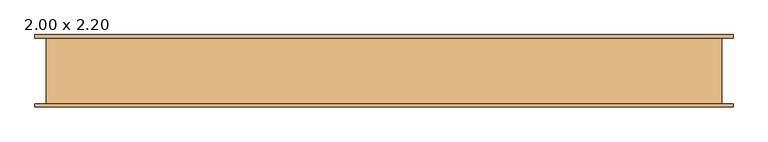
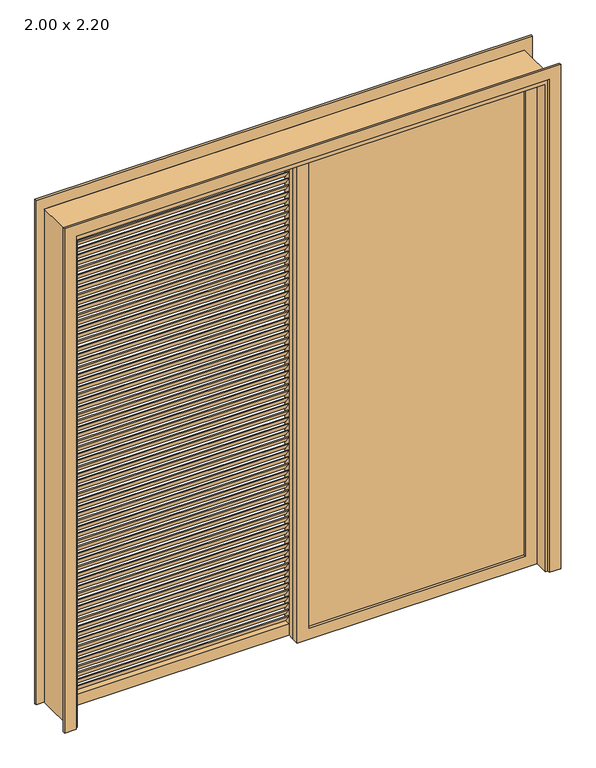
"""IFC4 building model written with IfcOpenShell, lengths in millimetres: door geometry, PORTA_DE_CORRER_3 FOLHAS_VENEZIANA_VIDRO : 2.00 x 2.20."""

from ifc_helpers import new_model, si_unit, frame, origin, place, context, project, spatial, polyline, outline, extrude, source, transform, mapped, element, save


def door_2_00_x_2_20_50220c9b(model_context):
    return source(origin(), model_context, "Body", "SweptSolid", [
        extrude(outline(polyline([(950.0, -26.0), (950.0, -34.0), (25.0, -34.0), (25.0, -26.0), (950.0, -26.0)])), frame((0.0, 0.0, 50.0), z_axis=(0.0, 0.0, 1.0), x_axis=(1.0, 0.0, 0.0)), (0.0, 0.0, 1.0), 2100.0),
        extrude(outline(polyline([(2200.0, 1000.0), (2200.0, -25.0), (0.0, -25.0), (0.0, 1000.0), (2200.0, 1000.0)]), holes=[polyline([(2150.0, 950.0), (50.0, 950.0), (50.0, 25.0), (2150.0, 25.0), (2150.0, 950.0)])]), frame((0.0, -45.0, 0.0), z_axis=(0.0, 1.0, 0.0), x_axis=(0.0, 0.0, 1.0)), (0.0, 0.0, 1.0), 30.0),
        extrude(outline(polyline([(40.0, 2085.0724638), (15.0, 2120.0724638), (20.0, 2120.0724638), (45.0, 2085.0724638), (40.0, 2085.0724638)])), frame((-950.0, 0.0, 0.0), z_axis=(1.0, 0.0, 0.0), x_axis=(0.0, 1.0, 0.0)), (0.0, 0.0, 1.0), 925.0),
        extrude(outline(polyline([(40.0, 2055.1449275), (15.0, 2090.1449275), (20.0, 2090.1449275), (45.0, 2055.1449275), (40.0, 2055.1449275)])), frame((-950.0, 0.0, 0.0), z_axis=(1.0, 0.0, 0.0), x_axis=(0.0, 1.0, 0.0)), (0.0, 0.0, 1.0), 925.0),
        extrude(outline(polyline([(40.0, 2025.2173913), (15.0, 2060.2173913), (20.0, 2060.2173913), (45.0, 2025.2173913), (40.0, 2025.2173913)])), frame((-950.0, 0.0, 0.0), z_axis=(1.0, 0.0, 0.0), x_axis=(0.0, 1.0, 0.0)), (0.0, 0.0, 1.0), 925.0),
        extrude(outline(polyline([(40.0, 1995.2898551), (15.0, 2030.2898551), (20.0, 2030.2898551), (45.0, 1995.2898551), (40.0, 1995.2898551)])), frame((-950.0, 0.0, 0.0), z_axis=(1.0, 0.0, 0.0), x_axis=(0.0, 1.0, 0.0)), (0.0, 0.0, 1.0), 925.0),
        extrude(outline(polyline([(40.0, 1965.3623188), (15.0, 2000.3623188), (20.0, 2000.3623188), (45.0, 1965.3623188), (40.0, 1965.3623188)])), frame((-950.0, 0.0, 0.0), z_axis=(1.0, 0.0, 0.0), x_axis=(0.0, 1.0, 0.0)), (0.0, 0.0, 1.0), 925.0),
        extrude(outline(polyline([(40.0, 1935.4347826), (15.0, 1970.4347826), (20.0, 1970.4347826), (45.0, 1935.4347826), (40.0, 1935.4347826)])), frame((-950.0, 0.0, 0.0), z_axis=(1.0, 0.0, 0.0), x_axis=(0.0, 1.0, 0.0)), (0.0, 0.0, 1.0), 925.0),
        extrude(outline(polyline([(40.0, 1905.5072464), (15.0, 1940.5072464), (20.0, 1940.5072464), (45.0, 1905.5072464), (40.0, 1905.5072464)])), frame((-950.0, 0.0, 0.0), z_axis=(1.0, 0.0, 0.0), x_axis=(0.0, 1.0, 0.0)), (0.0, 0.0, 1.0), 925.0),
        extrude(outline(polyline([(40.0, 1875.5797101), (15.0, 1910.5797101), (20.0, 1910.5797101), (45.0, 1875.5797101), (40.0, 1875.5797101)])), frame((-950.0, 0.0, 0.0), z_axis=(1.0, 0.0, 0.0), x_axis=(0.0, 1.0, 0.0)), (0.0, 0.0, 1.0), 925.0),
        extrude(outline(polyline([(40.0, 1845.6521739), (15.0, 1880.6521739), (20.0, 1880.6521739), (45.0, 1845.6521739), (40.0, 1845.6521739)])), frame((-950.0, 0.0, 0.0), z_axis=(1.0, 0.0, 0.0), x_axis=(0.0, 1.0, 0.0)), (0.0, 0.0, 1.0), 925.0),
        extrude(outline(polyline([(40.0, 1815.7246377), (15.0, 1850.7246377), (20.0, 1850.7246377), (45.0, 1815.7246377), (40.0, 1815.7246377)])), frame((-950.0, 0.0, 0.0), z_axis=(1.0, 0.0, 0.0), x_axis=(0.0, 1.0, 0.0)), (0.0, 0.0, 1.0), 925.0),
        extrude(outline(polyline([(40.0, 1785.7971014), (15.0, 1820.7971014), (20.0, 1820.7971014), (45.0, 1785.7971014), (40.0, 1785.7971014)])), frame((-950.0, 0.0, 0.0), z_axis=(1.0, 0.0, 0.0), x_axis=(0.0, 1.0, 0.0)), (0.0, 0.0, 1.0), 925.0),
        extrude(outline(polyline([(40.0, 1755.8695652), (15.0, 1790.8695652), (20.0, 1790.8695652), (45.0, 1755.8695652), (40.0, 1755.8695652)])), frame((-950.0, 0.0, 0.0), z_axis=(1.0, 0.0, 0.0), x_axis=(0.0, 1.0, 0.0)), (0.0, 0.0, 1.0), 925.0),
        extrude(outline(polyline([(40.0, 1725.942029), (15.0, 1760.942029), (20.0, 1760.942029), (45.0, 1725.942029), (40.0, 1725.942029)])), frame((-950.0, 0.0, 0.0), z_axis=(1.0, 0.0, 0.0), x_axis=(0.0, 1.0, 0.0)), (0.0, 0.0, 1.0), 925.0),
        extrude(outline(polyline([(40.0, 1696.0144928), (15.0, 1731.0144928), (20.0, 1731.0144928), (45.0, 1696.0144928), (40.0, 1696.0144928)])), frame((-950.0, 0.0, 0.0), z_axis=(1.0, 0.0, 0.0), x_axis=(0.0, 1.0, 0.0)), (0.0, 0.0, 1.0), 925.0),
        extrude(outline(polyline([(40.0, 1666.0869565), (15.0, 1701.0869565), (20.0, 1701.0869565), (45.0, 1666.0869565), (40.0, 1666.0869565)])), frame((-950.0, 0.0, 0.0), z_axis=(1.0, 0.0, 0.0), x_axis=(0.0, 1.0, 0.0)), (0.0, 0.0, 1.0), 925.0),
        extrude(outline(polyline([(40.0, 1636.1594203), (15.0, 1671.1594203), (20.0, 1671.1594203), (45.0, 1636.1594203), (40.0, 1636.1594203)])), frame((-950.0, 0.0, 0.0), z_axis=(1.0, 0.0, 0.0), x_axis=(0.0, 1.0, 0.0)), (0.0, 0.0, 1.0), 925.0),
        extrude(outline(polyline([(40.0, 1606.2318841), (15.0, 1641.2318841), (20.0, 1641.2318841), (45.0, 1606.2318841), (40.0, 1606.2318841)])), frame((-950.0, 0.0, 0.0), z_axis=(1.0, 0.0, 0.0), x_axis=(0.0, 1.0, 0.0)), (0.0, 0.0, 1.0), 925.0),
        extrude(outline(polyline([(40.0, 1576.3043478), (15.0, 1611.3043478), (20.0, 1611.3043478), (45.0, 1576.3043478), (40.0, 1576.3043478)])), frame((-950.0, 0.0, 0.0), z_axis=(1.0, 0.0, 0.0), x_axis=(0.0, 1.0, 0.0)), (0.0, 0.0, 1.0), 925.0),
        extrude(outline(polyline([(40.0, 1546.3768116), (15.0, 1581.3768116), (20.0, 1581.3768116), (45.0, 1546.3768116), (40.0, 1546.3768116)])), frame((-950.0, 0.0, 0.0), z_axis=(1.0, 0.0, 0.0), x_axis=(0.0, 1.0, 0.0)), (0.0, 0.0, 1.0), 925.0),
        extrude(outline(polyline([(40.0, 1516.4492754), (15.0, 1551.4492754), (20.0, 1551.4492754), (45.0, 1516.4492754), (40.0, 1516.4492754)])), frame((-950.0, 0.0, 0.0), z_axis=(1.0, 0.0, 0.0), x_axis=(0.0, 1.0, 0.0)), (0.0, 0.0, 1.0), 925.0),
        extrude(outline(polyline([(40.0, 1486.5217391), (15.0, 1521.5217391), (20.0, 1521.5217391), (45.0, 1486.5217391), (40.0, 1486.5217391)])), frame((-950.0, 0.0, 0.0), z_axis=(1.0, 0.0, 0.0), x_axis=(0.0, 1.0, 0.0)), (0.0, 0.0, 1.0), 925.0),
        extrude(outline(polyline([(40.0, 1456.5942029), (15.0, 1491.5942029), (20.0, 1491.5942029), (45.0, 1456.5942029), (40.0, 1456.5942029)])), frame((-950.0, 0.0, 0.0), z_axis=(1.0, 0.0, 0.0), x_axis=(0.0, 1.0, 0.0)), (0.0, 0.0, 1.0), 925.0),
        extrude(outline(polyline([(40.0, 1426.6666667), (15.0, 1461.6666667), (20.0, 1461.6666667), (45.0, 1426.6666667), (40.0, 1426.6666667)])), frame((-950.0, 0.0, 0.0), z_axis=(1.0, 0.0, 0.0), x_axis=(0.0, 1.0, 0.0)), (0.0, 0.0, 1.0), 925.0),
        extrude(outline(polyline([(40.0, 1396.7391304), (15.0, 1431.7391304), (20.0, 1431.7391304), (45.0, 1396.7391304), (40.0, 1396.7391304)])), frame((-950.0, 0.0, 0.0), z_axis=(1.0, 0.0, 0.0), x_axis=(0.0, 1.0, 0.0)), (0.0, 0.0, 1.0), 925.0),
        extrude(outline(polyline([(40.0, 1366.8115942), (15.0, 1401.8115942), (20.0, 1401.8115942), (45.0, 1366.8115942), (40.0, 1366.8115942)])), frame((-950.0, 0.0, 0.0), z_axis=(1.0, 0.0, 0.0), x_axis=(0.0, 1.0, 0.0)), (0.0, 0.0, 1.0), 925.0),
        extrude(outline(polyline([(40.0, 1336.884058), (15.0, 1371.884058), (20.0, 1371.884058), (45.0, 1336.884058), (40.0, 1336.884058)])), frame((-950.0, 0.0, 0.0), z_axis=(1.0, 0.0, 0.0), x_axis=(0.0, 1.0, 0.0)), (0.0, 0.0, 1.0), 925.0),
        extrude(outline(polyline([(40.0, 1306.9565217), (15.0, 1341.9565217), (20.0, 1341.9565217), (45.0, 1306.9565217), (40.0, 1306.9565217)])), frame((-950.0, 0.0, 0.0), z_axis=(1.0, 0.0, 0.0), x_axis=(0.0, 1.0, 0.0)), (0.0, 0.0, 1.0), 925.0),
        extrude(outline(polyline([(40.0, 1277.0289855), (15.0, 1312.0289855), (20.0, 1312.0289855), (45.0, 1277.0289855), (40.0, 1277.0289855)])), frame((-950.0, 0.0, 0.0), z_axis=(1.0, 0.0, 0.0), x_axis=(0.0, 1.0, 0.0)), (0.0, 0.0, 1.0), 925.0),
        extrude(outline(polyline([(40.0, 1247.1014493), (15.0, 1282.1014493), (20.0, 1282.1014493), (45.0, 1247.1014493), (40.0, 1247.1014493)])), frame((-950.0, 0.0, 0.0), z_axis=(1.0, 0.0, 0.0), x_axis=(0.0, 1.0, 0.0)), (0.0, 0.0, 1.0), 925.0),
        extrude(outline(polyline([(40.0, 1217.173913), (15.0, 1252.173913), (20.0, 1252.173913), (45.0, 1217.173913), (40.0, 1217.173913)])), frame((-950.0, 0.0, 0.0), z_axis=(1.0, 0.0, 0.0), x_axis=(0.0, 1.0, 0.0)), (0.0, 0.0, 1.0), 925.0),
        extrude(outline(polyline([(40.0, 1187.2463768), (15.0, 1222.2463768), (20.0, 1222.2463768), (45.0, 1187.2463768), (40.0, 1187.2463768)])), frame((-950.0, 0.0, 0.0), z_axis=(1.0, 0.0, 0.0), x_axis=(0.0, 1.0, 0.0)), (0.0, 0.0, 1.0), 925.0),
        extrude(outline(polyline([(40.0, 1157.3188406), (15.0, 1192.3188406), (20.0, 1192.3188406), (45.0, 1157.3188406), (40.0, 1157.3188406)])), frame((-950.0, 0.0, 0.0), z_axis=(1.0, 0.0, 0.0), x_axis=(0.0, 1.0, 0.0)), (0.0, 0.0, 1.0), 925.0),
        extrude(outline(polyline([(40.0, 1127.3913043), (15.0, 1162.3913043), (20.0, 1162.3913043), (45.0, 1127.3913043), (40.0, 1127.3913043)])), frame((-950.0, 0.0, 0.0), z_axis=(1.0, 0.0, 0.0), x_axis=(0.0, 1.0, 0.0)), (0.0, 0.0, 1.0), 925.0),
        extrude(outline(polyline([(40.0, 1097.4637681), (15.0, 1132.4637681), (20.0, 1132.4637681), (45.0, 1097.4637681), (40.0, 1097.4637681)])), frame((-950.0, 0.0, 0.0), z_axis=(1.0, 0.0, 0.0), x_axis=(0.0, 1.0, 0.0)), (0.0, 0.0, 1.0), 925.0),
        extrude(outline(polyline([(40.0, 1067.5362319), (15.0, 1102.5362319), (20.0, 1102.5362319), (45.0, 1067.5362319), (40.0, 1067.5362319)])), frame((-950.0, 0.0, 0.0), z_axis=(1.0, 0.0, 0.0), x_axis=(0.0, 1.0, 0.0)), (0.0, 0.0, 1.0), 925.0),
        extrude(outline(polyline([(40.0, 1037.6086957), (15.0, 1072.6086957), (20.0, 1072.6086957), (45.0, 1037.6086957), (40.0, 1037.6086957)])), frame((-950.0, 0.0, 0.0), z_axis=(1.0, 0.0, 0.0), x_axis=(0.0, 1.0, 0.0)), (0.0, 0.0, 1.0), 925.0),
        extrude(outline(polyline([(40.0, 1007.6811594), (15.0, 1042.6811594), (20.0, 1042.6811594), (45.0, 1007.6811594), (40.0, 1007.6811594)])), frame((-950.0, 0.0, 0.0), z_axis=(1.0, 0.0, 0.0), x_axis=(0.0, 1.0, 0.0)), (0.0, 0.0, 1.0), 925.0),
        extrude(outline(polyline([(40.0, 977.7536232), (15.0, 1012.7536232), (20.0, 1012.7536232), (45.0, 977.7536232), (40.0, 977.7536232)])), frame((-950.0, 0.0, 0.0), z_axis=(1.0, 0.0, 0.0), x_axis=(0.0, 1.0, 0.0)), (0.0, 0.0, 1.0), 925.0),
        extrude(outline(polyline([(40.0, 947.826087), (15.0, 982.826087), (20.0, 982.826087), (45.0, 947.826087), (40.0, 947.826087)])), frame((-950.0, 0.0, 0.0), z_axis=(1.0, 0.0, 0.0), x_axis=(0.0, 1.0, 0.0)), (0.0, 0.0, 1.0), 925.0),
        extrude(outline(polyline([(40.0, 917.8985507), (15.0, 952.8985507), (20.0, 952.8985507), (45.0, 917.8985507), (40.0, 917.8985507)])), frame((-950.0, 0.0, 0.0), z_axis=(1.0, 0.0, 0.0), x_axis=(0.0, 1.0, 0.0)), (0.0, 0.0, 1.0), 925.0),
        extrude(outline(polyline([(40.0, 887.9710145), (15.0, 922.9710145), (20.0, 922.9710145), (45.0, 887.9710145), (40.0, 887.9710145)])), frame((-950.0, 0.0, 0.0), z_axis=(1.0, 0.0, 0.0), x_axis=(0.0, 1.0, 0.0)), (0.0, 0.0, 1.0), 925.0),
        extrude(outline(polyline([(40.0, 858.0434783), (15.0, 893.0434783), (20.0, 893.0434783), (45.0, 858.0434783), (40.0, 858.0434783)])), frame((-950.0, 0.0, 0.0), z_axis=(1.0, 0.0, 0.0), x_axis=(0.0, 1.0, 0.0)), (0.0, 0.0, 1.0), 925.0),
        extrude(outline(polyline([(40.0, 828.115942), (15.0, 863.115942), (20.0, 863.115942), (45.0, 828.115942), (40.0, 828.115942)])), frame((-950.0, 0.0, 0.0), z_axis=(1.0, 0.0, 0.0), x_axis=(0.0, 1.0, 0.0)), (0.0, 0.0, 1.0), 925.0),
        extrude(outline(polyline([(40.0, 798.1884058), (15.0, 833.1884058), (20.0, 833.1884058), (45.0, 798.1884058), (40.0, 798.1884058)])), frame((-950.0, 0.0, 0.0), z_axis=(1.0, 0.0, 0.0), x_axis=(0.0, 1.0, 0.0)), (0.0, 0.0, 1.0), 925.0),
        extrude(outline(polyline([(40.0, 768.2608696), (15.0, 803.2608696), (20.0, 803.2608696), (45.0, 768.2608696), (40.0, 768.2608696)])), frame((-950.0, 0.0, 0.0), z_axis=(1.0, 0.0, 0.0), x_axis=(0.0, 1.0, 0.0)), (0.0, 0.0, 1.0), 925.0),
        extrude(outline(polyline([(40.0, 738.3333333), (15.0, 773.3333333), (20.0, 773.3333333), (45.0, 738.3333333), (40.0, 738.3333333)])), frame((-950.0, 0.0, 0.0), z_axis=(1.0, 0.0, 0.0), x_axis=(0.0, 1.0, 0.0)), (0.0, 0.0, 1.0), 925.0),
        extrude(outline(polyline([(40.0, 708.4057971), (15.0, 743.4057971), (20.0, 743.4057971), (45.0, 708.4057971), (40.0, 708.4057971)])), frame((-950.0, 0.0, 0.0), z_axis=(1.0, 0.0, 0.0), x_axis=(0.0, 1.0, 0.0)), (0.0, 0.0, 1.0), 925.0),
        extrude(outline(polyline([(40.0, 678.4782609), (15.0, 713.4782609), (20.0, 713.4782609), (45.0, 678.4782609), (40.0, 678.4782609)])), frame((-950.0, 0.0, 0.0), z_axis=(1.0, 0.0, 0.0), x_axis=(0.0, 1.0, 0.0)), (0.0, 0.0, 1.0), 925.0),
        extrude(outline(polyline([(40.0, 648.5507246), (15.0, 683.5507246), (20.0, 683.5507246), (45.0, 648.5507246), (40.0, 648.5507246)])), frame((-950.0, 0.0, 0.0), z_axis=(1.0, 0.0, 0.0), x_axis=(0.0, 1.0, 0.0)), (0.0, 0.0, 1.0), 925.0),
        extrude(outline(polyline([(40.0, 618.6231884), (15.0, 653.6231884), (20.0, 653.6231884), (45.0, 618.6231884), (40.0, 618.6231884)])), frame((-950.0, 0.0, 0.0), z_axis=(1.0, 0.0, 0.0), x_axis=(0.0, 1.0, 0.0)), (0.0, 0.0, 1.0), 925.0),
        extrude(outline(polyline([(40.0, 588.6956522), (15.0, 623.6956522), (20.0, 623.6956522), (45.0, 588.6956522), (40.0, 588.6956522)])), frame((-950.0, 0.0, 0.0), z_axis=(1.0, 0.0, 0.0), x_axis=(0.0, 1.0, 0.0)), (0.0, 0.0, 1.0), 925.0),
        extrude(outline(polyline([(40.0, 558.7681159), (15.0, 593.7681159), (20.0, 593.7681159), (45.0, 558.7681159), (40.0, 558.7681159)])), frame((-950.0, 0.0, 0.0), z_axis=(1.0, 0.0, 0.0), x_axis=(0.0, 1.0, 0.0)), (0.0, 0.0, 1.0), 925.0),
        extrude(outline(polyline([(40.0, 528.8405797), (15.0, 563.8405797), (20.0, 563.8405797), (45.0, 528.8405797), (40.0, 528.8405797)])), frame((-950.0, 0.0, 0.0), z_axis=(1.0, 0.0, 0.0), x_axis=(0.0, 1.0, 0.0)), (0.0, 0.0, 1.0), 925.0),
        extrude(outline(polyline([(40.0, 498.9130435), (15.0, 533.9130435), (20.0, 533.9130435), (45.0, 498.9130435), (40.0, 498.9130435)])), frame((-950.0, 0.0, 0.0), z_axis=(1.0, 0.0, 0.0), x_axis=(0.0, 1.0, 0.0)), (0.0, 0.0, 1.0), 925.0),
        extrude(outline(polyline([(40.0, 468.9855072), (15.0, 503.9855072), (20.0, 503.9855072), (45.0, 468.9855072), (40.0, 468.9855072)])), frame((-950.0, 0.0, 0.0), z_axis=(1.0, 0.0, 0.0), x_axis=(0.0, 1.0, 0.0)), (0.0, 0.0, 1.0), 925.0),
        extrude(outline(polyline([(40.0, 439.057971), (15.0, 474.057971), (20.0, 474.057971), (45.0, 439.057971), (40.0, 439.057971)])), frame((-950.0, 0.0, 0.0), z_axis=(1.0, 0.0, 0.0), x_axis=(0.0, 1.0, 0.0)), (0.0, 0.0, 1.0), 925.0),
        extrude(outline(polyline([(40.0, 409.1304348), (15.0, 444.1304348), (20.0, 444.1304348), (45.0, 409.1304348), (40.0, 409.1304348)])), frame((-950.0, 0.0, 0.0), z_axis=(1.0, 0.0, 0.0), x_axis=(0.0, 1.0, 0.0)), (0.0, 0.0, 1.0), 925.0),
        extrude(outline(polyline([(40.0, 379.2028986), (15.0, 414.2028986), (20.0, 414.2028986), (45.0, 379.2028986), (40.0, 379.2028986)])), frame((-950.0, 0.0, 0.0), z_axis=(1.0, 0.0, 0.0), x_axis=(0.0, 1.0, 0.0)), (0.0, 0.0, 1.0), 925.0),
        extrude(outline(polyline([(40.0, 349.2753623), (15.0, 384.2753623), (20.0, 384.2753623), (45.0, 349.2753623), (40.0, 349.2753623)])), frame((-950.0, 0.0, 0.0), z_axis=(1.0, 0.0, 0.0), x_axis=(0.0, 1.0, 0.0)), (0.0, 0.0, 1.0), 925.0),
        extrude(outline(polyline([(40.0, 319.3478261), (15.0, 354.3478261), (20.0, 354.3478261), (45.0, 319.3478261), (40.0, 319.3478261)])), frame((-950.0, 0.0, 0.0), z_axis=(1.0, 0.0, 0.0), x_axis=(0.0, 1.0, 0.0)), (0.0, 0.0, 1.0), 925.0),
        extrude(outline(polyline([(40.0, 289.4202899), (15.0, 324.4202899), (20.0, 324.4202899), (45.0, 289.4202899), (40.0, 289.4202899)])), frame((-950.0, 0.0, 0.0), z_axis=(1.0, 0.0, 0.0), x_axis=(0.0, 1.0, 0.0)), (0.0, 0.0, 1.0), 925.0),
        extrude(outline(polyline([(40.0, 259.4927536), (15.0, 294.4927536), (20.0, 294.4927536), (45.0, 259.4927536), (40.0, 259.4927536)])), frame((-950.0, 0.0, 0.0), z_axis=(1.0, 0.0, 0.0), x_axis=(0.0, 1.0, 0.0)), (0.0, 0.0, 1.0), 925.0),
        extrude(outline(polyline([(40.0, 229.5652174), (15.0, 264.5652174), (20.0, 264.5652174), (45.0, 229.5652174), (40.0, 229.5652174)])), frame((-950.0, 0.0, 0.0), z_axis=(1.0, 0.0, 0.0), x_axis=(0.0, 1.0, 0.0)), (0.0, 0.0, 1.0), 925.0),
        extrude(outline(polyline([(40.0, 199.6376812), (15.0, 234.6376812), (20.0, 234.6376812), (45.0, 199.6376812), (40.0, 199.6376812)])), frame((-950.0, 0.0, 0.0), z_axis=(1.0, 0.0, 0.0), x_axis=(0.0, 1.0, 0.0)), (0.0, 0.0, 1.0), 925.0),
        extrude(outline(polyline([(40.0, 169.7101449), (15.0, 204.7101449), (20.0, 204.7101449), (45.0, 169.7101449), (40.0, 169.7101449)])), frame((-950.0, 0.0, 0.0), z_axis=(1.0, 0.0, 0.0), x_axis=(0.0, 1.0, 0.0)), (0.0, 0.0, 1.0), 925.0),
        extrude(outline(polyline([(40.0, 139.7826087), (15.0, 174.7826087), (20.0, 174.7826087), (45.0, 139.7826087), (40.0, 139.7826087)])), frame((-950.0, 0.0, 0.0), z_axis=(1.0, 0.0, 0.0), x_axis=(0.0, 1.0, 0.0)), (0.0, 0.0, 1.0), 925.0),
        extrude(outline(polyline([(40.0, 109.8550725), (15.0, 144.8550725), (20.0, 144.8550725), (45.0, 109.8550725), (40.0, 109.8550725)])), frame((-950.0, 0.0, 0.0), z_axis=(1.0, 0.0, 0.0), x_axis=(0.0, 1.0, 0.0)), (0.0, 0.0, 1.0), 925.0),
        extrude(outline(polyline([(40.0, 79.9275362), (15.0, 114.9275362), (20.0, 114.9275362), (45.0, 79.9275362), (40.0, 79.9275362)])), frame((-950.0, 0.0, 0.0), z_axis=(1.0, 0.0, 0.0), x_axis=(0.0, 1.0, 0.0)), (0.0, 0.0, 1.0), 925.0),
        extrude(outline(polyline([(40.0, 2115.0), (15.0, 2150.0), (20.0, 2150.0), (45.0, 2115.0), (40.0, 2115.0)])), frame((-950.0, 0.0, 0.0), z_axis=(1.0, 0.0, 0.0), x_axis=(0.0, 1.0, 0.0)), (0.0, 0.0, 1.0), 925.0),
        extrude(outline(polyline([(40.0, 50.0), (15.0, 85.0), (20.0, 85.0), (45.0, 50.0), (40.0, 50.0)])), frame((-950.0, 0.0, 0.0), z_axis=(1.0, 0.0, 0.0), x_axis=(0.0, 1.0, 0.0)), (0.0, 0.0, 1.0), 925.0),
        extrude(outline(polyline([(2200.0, 25.0), (2200.0, -1000.0), (0.0, -1000.0), (0.0, 25.0), (2200.0, 25.0)]), holes=[polyline([(2150.0, -25.0), (50.0, -25.0), (50.0, -950.0), (2150.0, -950.0), (2150.0, -25.0)])]), frame((0.0, 15.0, 0.0), z_axis=(0.0, 1.0, 0.0), x_axis=(0.0, 0.0, 1.0)), (0.0, 0.0, 1.0), 30.0),
        extrude(outline(polyline([(10.0, 2085.0724638), (-15.0, 2120.0724638), (-10.0, 2120.0724638), (15.0, 2085.0724638), (10.0, 2085.0724638)])), frame((25.0, 0.0, 0.0), z_axis=(1.0, 0.0, 0.0), x_axis=(0.0, 1.0, 0.0)), (0.0, 0.0, 1.0), 925.0),
        extrude(outline(polyline([(10.0, 2055.1449275), (-15.0, 2090.1449275), (-10.0, 2090.1449275), (15.0, 2055.1449275), (10.0, 2055.1449275)])), frame((25.0, 0.0, 0.0), z_axis=(1.0, 0.0, 0.0), x_axis=(0.0, 1.0, 0.0)), (0.0, 0.0, 1.0), 925.0),
        extrude(outline(polyline([(10.0, 2025.2173913), (-15.0, 2060.2173913), (-10.0, 2060.2173913), (15.0, 2025.2173913), (10.0, 2025.2173913)])), frame((25.0, 0.0, 0.0), z_axis=(1.0, 0.0, 0.0), x_axis=(0.0, 1.0, 0.0)), (0.0, 0.0, 1.0), 925.0),
        extrude(outline(polyline([(10.0, 1995.2898551), (-15.0, 2030.2898551), (-10.0, 2030.2898551), (15.0, 1995.2898551), (10.0, 1995.2898551)])), frame((25.0, 0.0, 0.0), z_axis=(1.0, 0.0, 0.0), x_axis=(0.0, 1.0, 0.0)), (0.0, 0.0, 1.0), 925.0),
        extrude(outline(polyline([(10.0, 1965.3623188), (-15.0, 2000.3623188), (-10.0, 2000.3623188), (15.0, 1965.3623188), (10.0, 1965.3623188)])), frame((25.0, 0.0, 0.0), z_axis=(1.0, 0.0, 0.0), x_axis=(0.0, 1.0, 0.0)), (0.0, 0.0, 1.0), 925.0),
        extrude(outline(polyline([(10.0, 1935.4347826), (-15.0, 1970.4347826), (-10.0, 1970.4347826), (15.0, 1935.4347826), (10.0, 1935.4347826)])), frame((25.0, 0.0, 0.0), z_axis=(1.0, 0.0, 0.0), x_axis=(0.0, 1.0, 0.0)), (0.0, 0.0, 1.0), 925.0),
        extrude(outline(polyline([(10.0, 1905.5072464), (-15.0, 1940.5072464), (-10.0, 1940.5072464), (15.0, 1905.5072464), (10.0, 1905.5072464)])), frame((25.0, 0.0, 0.0), z_axis=(1.0, 0.0, 0.0), x_axis=(0.0, 1.0, 0.0)), (0.0, 0.0, 1.0), 925.0),
        extrude(outline(polyline([(10.0, 1875.5797101), (-15.0, 1910.5797101), (-10.0, 1910.5797101), (15.0, 1875.5797101), (10.0, 1875.5797101)])), frame((25.0, 0.0, 0.0), z_axis=(1.0, 0.0, 0.0), x_axis=(0.0, 1.0, 0.0)), (0.0, 0.0, 1.0), 925.0),
        extrude(outline(polyline([(10.0, 1845.6521739), (-15.0, 1880.6521739), (-10.0, 1880.6521739), (15.0, 1845.6521739), (10.0, 1845.6521739)])), frame((25.0, 0.0, 0.0), z_axis=(1.0, 0.0, 0.0), x_axis=(0.0, 1.0, 0.0)), (0.0, 0.0, 1.0), 925.0),
        extrude(outline(polyline([(10.0, 1815.7246377), (-15.0, 1850.7246377), (-10.0, 1850.7246377), (15.0, 1815.7246377), (10.0, 1815.7246377)])), frame((25.0, 0.0, 0.0), z_axis=(1.0, 0.0, 0.0), x_axis=(0.0, 1.0, 0.0)), (0.0, 0.0, 1.0), 925.0),
        extrude(outline(polyline([(10.0, 1785.7971014), (-15.0, 1820.7971014), (-10.0, 1820.7971014), (15.0, 1785.7971014), (10.0, 1785.7971014)])), frame((25.0, 0.0, 0.0), z_axis=(1.0, 0.0, 0.0), x_axis=(0.0, 1.0, 0.0)), (0.0, 0.0, 1.0), 925.0),
        extrude(outline(polyline([(10.0, 1755.8695652), (-15.0, 1790.8695652), (-10.0, 1790.8695652), (15.0, 1755.8695652), (10.0, 1755.8695652)])), frame((25.0, 0.0, 0.0), z_axis=(1.0, 0.0, 0.0), x_axis=(0.0, 1.0, 0.0)), (0.0, 0.0, 1.0), 925.0),
        extrude(outline(polyline([(10.0, 1725.942029), (-15.0, 1760.942029), (-10.0, 1760.942029), (15.0, 1725.942029), (10.0, 1725.942029)])), frame((25.0, 0.0, 0.0), z_axis=(1.0, 0.0, 0.0), x_axis=(0.0, 1.0, 0.0)), (0.0, 0.0, 1.0), 925.0),
        extrude(outline(polyline([(10.0, 1696.0144928), (-15.0, 1731.0144928), (-10.0, 1731.0144928), (15.0, 1696.0144928), (10.0, 1696.0144928)])), frame((25.0, 0.0, 0.0), z_axis=(1.0, 0.0, 0.0), x_axis=(0.0, 1.0, 0.0)), (0.0, 0.0, 1.0), 925.0),
        extrude(outline(polyline([(10.0, 1666.0869565), (-15.0, 1701.0869565), (-10.0, 1701.0869565), (15.0, 1666.0869565), (10.0, 1666.0869565)])), frame((25.0, 0.0, 0.0), z_axis=(1.0, 0.0, 0.0), x_axis=(0.0, 1.0, 0.0)), (0.0, 0.0, 1.0), 925.0),
        extrude(outline(polyline([(10.0, 1636.1594203), (-15.0, 1671.1594203), (-10.0, 1671.1594203), (15.0, 1636.1594203), (10.0, 1636.1594203)])), frame((25.0, 0.0, 0.0), z_axis=(1.0, 0.0, 0.0), x_axis=(0.0, 1.0, 0.0)), (0.0, 0.0, 1.0), 925.0),
        extrude(outline(polyline([(10.0, 1606.2318841), (-15.0, 1641.2318841), (-10.0, 1641.2318841), (15.0, 1606.2318841), (10.0, 1606.2318841)])), frame((25.0, 0.0, 0.0), z_axis=(1.0, 0.0, 0.0), x_axis=(0.0, 1.0, 0.0)), (0.0, 0.0, 1.0), 925.0),
        extrude(outline(polyline([(10.0, 1576.3043478), (-15.0, 1611.3043478), (-10.0, 1611.3043478), (15.0, 1576.3043478), (10.0, 1576.3043478)])), frame((25.0, 0.0, 0.0), z_axis=(1.0, 0.0, 0.0), x_axis=(0.0, 1.0, 0.0)), (0.0, 0.0, 1.0), 925.0),
        extrude(outline(polyline([(10.0, 1546.3768116), (-15.0, 1581.3768116), (-10.0, 1581.3768116), (15.0, 1546.3768116), (10.0, 1546.3768116)])), frame((25.0, 0.0, 0.0), z_axis=(1.0, 0.0, 0.0), x_axis=(0.0, 1.0, 0.0)), (0.0, 0.0, 1.0), 925.0),
        extrude(outline(polyline([(10.0, 1516.4492754), (-15.0, 1551.4492754), (-10.0, 1551.4492754), (15.0, 1516.4492754), (10.0, 1516.4492754)])), frame((25.0, 0.0, 0.0), z_axis=(1.0, 0.0, 0.0), x_axis=(0.0, 1.0, 0.0)), (0.0, 0.0, 1.0), 925.0),
        extrude(outline(polyline([(10.0, 1486.5217391), (-15.0, 1521.5217391), (-10.0, 1521.5217391), (15.0, 1486.5217391), (10.0, 1486.5217391)])), frame((25.0, 0.0, 0.0), z_axis=(1.0, 0.0, 0.0), x_axis=(0.0, 1.0, 0.0)), (0.0, 0.0, 1.0), 925.0),
        extrude(outline(polyline([(10.0, 1456.5942029), (-15.0, 1491.5942029), (-10.0, 1491.5942029), (15.0, 1456.5942029), (10.0, 1456.5942029)])), frame((25.0, 0.0, 0.0), z_axis=(1.0, 0.0, 0.0), x_axis=(0.0, 1.0, 0.0)), (0.0, 0.0, 1.0), 925.0),
        extrude(outline(polyline([(10.0, 1426.6666667), (-15.0, 1461.6666667), (-10.0, 1461.6666667), (15.0, 1426.6666667), (10.0, 1426.6666667)])), frame((25.0, 0.0, 0.0), z_axis=(1.0, 0.0, 0.0), x_axis=(0.0, 1.0, 0.0)), (0.0, 0.0, 1.0), 925.0),
        extrude(outline(polyline([(10.0, 1396.7391304), (-15.0, 1431.7391304), (-10.0, 1431.7391304), (15.0, 1396.7391304), (10.0, 1396.7391304)])), frame((25.0, 0.0, 0.0), z_axis=(1.0, 0.0, 0.0), x_axis=(0.0, 1.0, 0.0)), (0.0, 0.0, 1.0), 925.0),
        extrude(outline(polyline([(10.0, 1366.8115942), (-15.0, 1401.8115942), (-10.0, 1401.8115942), (15.0, 1366.8115942), (10.0, 1366.8115942)])), frame((25.0, 0.0, 0.0), z_axis=(1.0, 0.0, 0.0), x_axis=(0.0, 1.0, 0.0)), (0.0, 0.0, 1.0), 925.0),
        extrude(outline(polyline([(10.0, 1336.884058), (-15.0, 1371.884058), (-10.0, 1371.884058), (15.0, 1336.884058), (10.0, 1336.884058)])), frame((25.0, 0.0, 0.0), z_axis=(1.0, 0.0, 0.0), x_axis=(0.0, 1.0, 0.0)), (0.0, 0.0, 1.0), 925.0),
        extrude(outline(polyline([(10.0, 1306.9565217), (-15.0, 1341.9565217), (-10.0, 1341.9565217), (15.0, 1306.9565217), (10.0, 1306.9565217)])), frame((25.0, 0.0, 0.0), z_axis=(1.0, 0.0, 0.0), x_axis=(0.0, 1.0, 0.0)), (0.0, 0.0, 1.0), 925.0),
        extrude(outline(polyline([(10.0, 1277.0289855), (-15.0, 1312.0289855), (-10.0, 1312.0289855), (15.0, 1277.0289855), (10.0, 1277.0289855)])), frame((25.0, 0.0, 0.0), z_axis=(1.0, 0.0, 0.0), x_axis=(0.0, 1.0, 0.0)), (0.0, 0.0, 1.0), 925.0),
        extrude(outline(polyline([(10.0, 1247.1014493), (-15.0, 1282.1014493), (-10.0, 1282.1014493), (15.0, 1247.1014493), (10.0, 1247.1014493)])), frame((25.0, 0.0, 0.0), z_axis=(1.0, 0.0, 0.0), x_axis=(0.0, 1.0, 0.0)), (0.0, 0.0, 1.0), 925.0),
        extrude(outline(polyline([(10.0, 1217.173913), (-15.0, 1252.173913), (-10.0, 1252.173913), (15.0, 1217.173913), (10.0, 1217.173913)])), frame((25.0, 0.0, 0.0), z_axis=(1.0, 0.0, 0.0), x_axis=(0.0, 1.0, 0.0)), (0.0, 0.0, 1.0), 925.0),
        extrude(outline(polyline([(10.0, 1187.2463768), (-15.0, 1222.2463768), (-10.0, 1222.2463768), (15.0, 1187.2463768), (10.0, 1187.2463768)])), frame((25.0, 0.0, 0.0), z_axis=(1.0, 0.0, 0.0), x_axis=(0.0, 1.0, 0.0)), (0.0, 0.0, 1.0), 925.0),
        extrude(outline(polyline([(10.0, 1157.3188406), (-15.0, 1192.3188406), (-10.0, 1192.3188406), (15.0, 1157.3188406), (10.0, 1157.3188406)])), frame((25.0, 0.0, 0.0), z_axis=(1.0, 0.0, 0.0), x_axis=(0.0, 1.0, 0.0)), (0.0, 0.0, 1.0), 925.0),
        extrude(outline(polyline([(10.0, 1127.3913043), (-15.0, 1162.3913043), (-10.0, 1162.3913043), (15.0, 1127.3913043), (10.0, 1127.3913043)])), frame((25.0, 0.0, 0.0), z_axis=(1.0, 0.0, 0.0), x_axis=(0.0, 1.0, 0.0)), (0.0, 0.0, 1.0), 925.0),
        extrude(outline(polyline([(10.0, 1097.4637681), (-15.0, 1132.4637681), (-10.0, 1132.4637681), (15.0, 1097.4637681), (10.0, 1097.4637681)])), frame((25.0, 0.0, 0.0), z_axis=(1.0, 0.0, 0.0), x_axis=(0.0, 1.0, 0.0)), (0.0, 0.0, 1.0), 925.0),
        extrude(outline(polyline([(10.0, 1067.5362319), (-15.0, 1102.5362319), (-10.0, 1102.5362319), (15.0, 1067.5362319), (10.0, 1067.5362319)])), frame((25.0, 0.0, 0.0), z_axis=(1.0, 0.0, 0.0), x_axis=(0.0, 1.0, 0.0)), (0.0, 0.0, 1.0), 925.0),
        extrude(outline(polyline([(10.0, 1037.6086957), (-15.0, 1072.6086957), (-10.0, 1072.6086957), (15.0, 1037.6086957), (10.0, 1037.6086957)])), frame((25.0, 0.0, 0.0), z_axis=(1.0, 0.0, 0.0), x_axis=(0.0, 1.0, 0.0)), (0.0, 0.0, 1.0), 925.0),
        extrude(outline(polyline([(10.0, 1007.6811594), (-15.0, 1042.6811594), (-10.0, 1042.6811594), (15.0, 1007.6811594), (10.0, 1007.6811594)])), frame((25.0, 0.0, 0.0), z_axis=(1.0, 0.0, 0.0), x_axis=(0.0, 1.0, 0.0)), (0.0, 0.0, 1.0), 925.0),
        extrude(outline(polyline([(10.0, 977.7536232), (-15.0, 1012.7536232), (-10.0, 1012.7536232), (15.0, 977.7536232), (10.0, 977.7536232)])), frame((25.0, 0.0, 0.0), z_axis=(1.0, 0.0, 0.0), x_axis=(0.0, 1.0, 0.0)), (0.0, 0.0, 1.0), 925.0),
        extrude(outline(polyline([(10.0, 947.826087), (-15.0, 982.826087), (-10.0, 982.826087), (15.0, 947.826087), (10.0, 947.826087)])), frame((25.0, 0.0, 0.0), z_axis=(1.0, 0.0, 0.0), x_axis=(0.0, 1.0, 0.0)), (0.0, 0.0, 1.0), 925.0),
        extrude(outline(polyline([(10.0, 917.8985507), (-15.0, 952.8985507), (-10.0, 952.8985507), (15.0, 917.8985507), (10.0, 917.8985507)])), frame((25.0, 0.0, 0.0), z_axis=(1.0, 0.0, 0.0), x_axis=(0.0, 1.0, 0.0)), (0.0, 0.0, 1.0), 925.0),
        extrude(outline(polyline([(10.0, 887.9710145), (-15.0, 922.9710145), (-10.0, 922.9710145), (15.0, 887.9710145), (10.0, 887.9710145)])), frame((25.0, 0.0, 0.0), z_axis=(1.0, 0.0, 0.0), x_axis=(0.0, 1.0, 0.0)), (0.0, 0.0, 1.0), 925.0),
        extrude(outline(polyline([(10.0, 858.0434783), (-15.0, 893.0434783), (-10.0, 893.0434783), (15.0, 858.0434783), (10.0, 858.0434783)])), frame((25.0, 0.0, 0.0), z_axis=(1.0, 0.0, 0.0), x_axis=(0.0, 1.0, 0.0)), (0.0, 0.0, 1.0), 925.0),
        extrude(outline(polyline([(10.0, 828.115942), (-15.0, 863.115942), (-10.0, 863.115942), (15.0, 828.115942), (10.0, 828.115942)])), frame((25.0, 0.0, 0.0), z_axis=(1.0, 0.0, 0.0), x_axis=(0.0, 1.0, 0.0)), (0.0, 0.0, 1.0), 925.0),
        extrude(outline(polyline([(10.0, 798.1884058), (-15.0, 833.1884058), (-10.0, 833.1884058), (15.0, 798.1884058), (10.0, 798.1884058)])), frame((25.0, 0.0, 0.0), z_axis=(1.0, 0.0, 0.0), x_axis=(0.0, 1.0, 0.0)), (0.0, 0.0, 1.0), 925.0),
        extrude(outline(polyline([(10.0, 768.2608696), (-15.0, 803.2608696), (-10.0, 803.2608696), (15.0, 768.2608696), (10.0, 768.2608696)])), frame((25.0, 0.0, 0.0), z_axis=(1.0, 0.0, 0.0), x_axis=(0.0, 1.0, 0.0)), (0.0, 0.0, 1.0), 925.0),
        extrude(outline(polyline([(10.0, 738.3333333), (-15.0, 773.3333333), (-10.0, 773.3333333), (15.0, 738.3333333), (10.0, 738.3333333)])), frame((25.0, 0.0, 0.0), z_axis=(1.0, 0.0, 0.0), x_axis=(0.0, 1.0, 0.0)), (0.0, 0.0, 1.0), 925.0),
        extrude(outline(polyline([(10.0, 708.4057971), (-15.0, 743.4057971), (-10.0, 743.4057971), (15.0, 708.4057971), (10.0, 708.4057971)])), frame((25.0, 0.0, 0.0), z_axis=(1.0, 0.0, 0.0), x_axis=(0.0, 1.0, 0.0)), (0.0, 0.0, 1.0), 925.0),
        extrude(outline(polyline([(10.0, 678.4782609), (-15.0, 713.4782609), (-10.0, 713.4782609), (15.0, 678.4782609), (10.0, 678.4782609)])), frame((25.0, 0.0, 0.0), z_axis=(1.0, 0.0, 0.0), x_axis=(0.0, 1.0, 0.0)), (0.0, 0.0, 1.0), 925.0),
        extrude(outline(polyline([(10.0, 648.5507246), (-15.0, 683.5507246), (-10.0, 683.5507246), (15.0, 648.5507246), (10.0, 648.5507246)])), frame((25.0, 0.0, 0.0), z_axis=(1.0, 0.0, 0.0), x_axis=(0.0, 1.0, 0.0)), (0.0, 0.0, 1.0), 925.0),
        extrude(outline(polyline([(10.0, 618.6231884), (-15.0, 653.6231884), (-10.0, 653.6231884), (15.0, 618.6231884), (10.0, 618.6231884)])), frame((25.0, 0.0, 0.0), z_axis=(1.0, 0.0, 0.0), x_axis=(0.0, 1.0, 0.0)), (0.0, 0.0, 1.0), 925.0),
        extrude(outline(polyline([(10.0, 588.6956522), (-15.0, 623.6956522), (-10.0, 623.6956522), (15.0, 588.6956522), (10.0, 588.6956522)])), frame((25.0, 0.0, 0.0), z_axis=(1.0, 0.0, 0.0), x_axis=(0.0, 1.0, 0.0)), (0.0, 0.0, 1.0), 925.0),
        extrude(outline(polyline([(10.0, 558.7681159), (-15.0, 593.7681159), (-10.0, 593.7681159), (15.0, 558.7681159), (10.0, 558.7681159)])), frame((25.0, 0.0, 0.0), z_axis=(1.0, 0.0, 0.0), x_axis=(0.0, 1.0, 0.0)), (0.0, 0.0, 1.0), 925.0),
        extrude(outline(polyline([(10.0, 528.8405797), (-15.0, 563.8405797), (-10.0, 563.8405797), (15.0, 528.8405797), (10.0, 528.8405797)])), frame((25.0, 0.0, 0.0), z_axis=(1.0, 0.0, 0.0), x_axis=(0.0, 1.0, 0.0)), (0.0, 0.0, 1.0), 925.0),
        extrude(outline(polyline([(10.0, 498.9130435), (-15.0, 533.9130435), (-10.0, 533.9130435), (15.0, 498.9130435), (10.0, 498.9130435)])), frame((25.0, 0.0, 0.0), z_axis=(1.0, 0.0, 0.0), x_axis=(0.0, 1.0, 0.0)), (0.0, 0.0, 1.0), 925.0),
        extrude(outline(polyline([(10.0, 468.9855072), (-15.0, 503.9855072), (-10.0, 503.9855072), (15.0, 468.9855072), (10.0, 468.9855072)])), frame((25.0, 0.0, 0.0), z_axis=(1.0, 0.0, 0.0), x_axis=(0.0, 1.0, 0.0)), (0.0, 0.0, 1.0), 925.0),
        extrude(outline(polyline([(10.0, 439.057971), (-15.0, 474.057971), (-10.0, 474.057971), (15.0, 439.057971), (10.0, 439.057971)])), frame((25.0, 0.0, 0.0), z_axis=(1.0, 0.0, 0.0), x_axis=(0.0, 1.0, 0.0)), (0.0, 0.0, 1.0), 925.0),
        extrude(outline(polyline([(10.0, 409.1304348), (-15.0, 444.1304348), (-10.0, 444.1304348), (15.0, 409.1304348), (10.0, 409.1304348)])), frame((25.0, 0.0, 0.0), z_axis=(1.0, 0.0, 0.0), x_axis=(0.0, 1.0, 0.0)), (0.0, 0.0, 1.0), 925.0),
        extrude(outline(polyline([(10.0, 379.2028986), (-15.0, 414.2028986), (-10.0, 414.2028986), (15.0, 379.2028986), (10.0, 379.2028986)])), frame((25.0, 0.0, 0.0), z_axis=(1.0, 0.0, 0.0), x_axis=(0.0, 1.0, 0.0)), (0.0, 0.0, 1.0), 925.0),
        extrude(outline(polyline([(10.0, 349.2753623), (-15.0, 384.2753623), (-10.0, 384.2753623), (15.0, 349.2753623), (10.0, 349.2753623)])), frame((25.0, 0.0, 0.0), z_axis=(1.0, 0.0, 0.0), x_axis=(0.0, 1.0, 0.0)), (0.0, 0.0, 1.0), 925.0),
        extrude(outline(polyline([(10.0, 319.3478261), (-15.0, 354.3478261), (-10.0, 354.3478261), (15.0, 319.3478261), (10.0, 319.3478261)])), frame((25.0, 0.0, 0.0), z_axis=(1.0, 0.0, 0.0), x_axis=(0.0, 1.0, 0.0)), (0.0, 0.0, 1.0), 925.0),
        extrude(outline(polyline([(10.0, 289.4202899), (-15.0, 324.4202899), (-10.0, 324.4202899), (15.0, 289.4202899), (10.0, 289.4202899)])), frame((25.0, 0.0, 0.0), z_axis=(1.0, 0.0, 0.0), x_axis=(0.0, 1.0, 0.0)), (0.0, 0.0, 1.0), 925.0),
        extrude(outline(polyline([(10.0, 259.4927536), (-15.0, 294.4927536), (-10.0, 294.4927536), (15.0, 259.4927536), (10.0, 259.4927536)])), frame((25.0, 0.0, 0.0), z_axis=(1.0, 0.0, 0.0), x_axis=(0.0, 1.0, 0.0)), (0.0, 0.0, 1.0), 925.0),
        extrude(outline(polyline([(10.0, 229.5652174), (-15.0, 264.5652174), (-10.0, 264.5652174), (15.0, 229.5652174), (10.0, 229.5652174)])), frame((25.0, 0.0, 0.0), z_axis=(1.0, 0.0, 0.0), x_axis=(0.0, 1.0, 0.0)), (0.0, 0.0, 1.0), 925.0),
        extrude(outline(polyline([(10.0, 199.6376812), (-15.0, 234.6376812), (-10.0, 234.6376812), (15.0, 199.6376812), (10.0, 199.6376812)])), frame((25.0, 0.0, 0.0), z_axis=(1.0, 0.0, 0.0), x_axis=(0.0, 1.0, 0.0)), (0.0, 0.0, 1.0), 925.0),
        extrude(outline(polyline([(10.0, 169.7101449), (-15.0, 204.7101449), (-10.0, 204.7101449), (15.0, 169.7101449), (10.0, 169.7101449)])), frame((25.0, 0.0, 0.0), z_axis=(1.0, 0.0, 0.0), x_axis=(0.0, 1.0, 0.0)), (0.0, 0.0, 1.0), 925.0),
        extrude(outline(polyline([(10.0, 139.7826087), (-15.0, 174.7826087), (-10.0, 174.7826087), (15.0, 139.7826087), (10.0, 139.7826087)])), frame((25.0, 0.0, 0.0), z_axis=(1.0, 0.0, 0.0), x_axis=(0.0, 1.0, 0.0)), (0.0, 0.0, 1.0), 925.0),
        extrude(outline(polyline([(10.0, 109.8550725), (-15.0, 144.8550725), (-10.0, 144.8550725), (15.0, 109.8550725), (10.0, 109.8550725)])), frame((25.0, 0.0, 0.0), z_axis=(1.0, 0.0, 0.0), x_axis=(0.0, 1.0, 0.0)), (0.0, 0.0, 1.0), 925.0),
        extrude(outline(polyline([(10.0, 79.9275362), (-15.0, 114.9275362), (-10.0, 114.9275362), (15.0, 79.9275362), (10.0, 79.9275362)])), frame((25.0, 0.0, 0.0), z_axis=(1.0, 0.0, 0.0), x_axis=(0.0, 1.0, 0.0)), (0.0, 0.0, 1.0), 925.0),
        extrude(outline(polyline([(10.0, 2115.0), (-15.0, 2150.0), (-10.0, 2150.0), (15.0, 2115.0), (10.0, 2115.0)])), frame((25.0, 0.0, 0.0), z_axis=(1.0, 0.0, 0.0), x_axis=(0.0, 1.0, 0.0)), (0.0, 0.0, 1.0), 925.0),
        extrude(outline(polyline([(10.0, 50.0), (-15.0, 85.0), (-10.0, 85.0), (15.0, 50.0), (10.0, 50.0)])), frame((25.0, 0.0, 0.0), z_axis=(1.0, 0.0, 0.0), x_axis=(0.0, 1.0, 0.0)), (0.0, 0.0, 1.0), 925.0),
        extrude(outline(polyline([(2200.0, 1000.0), (2200.0, -25.0), (0.0, -25.0), (0.0, 1000.0), (2200.0, 1000.0)]), holes=[polyline([(2150.0, 950.0), (50.0, 950.0), (50.0, 25.0), (2150.0, 25.0), (2150.0, 950.0)])]), frame((0.0, -15.0, 0.0), z_axis=(0.0, 1.0, 0.0), x_axis=(0.0, 0.0, 1.0)), (0.0, 0.0, 1.0), 30.0),
        extrude(outline(polyline([(0.0, 1010.0), (0.0, 1060.0), (2275.0, 1060.0), (2275.0, -1060.0), (0.0, -1060.0), (0.0, -1010.0), (2225.0, -1010.0), (2225.0, 1010.0), (0.0, 1010.0)])), frame((0.0, 92.5, 0.0), z_axis=(0.0, 1.0, 0.0), x_axis=(0.0, 0.0, 1.0)), (0.0, 0.0, 1.0), 10.0),
        extrude(outline(polyline([(0.0, -1060.0), (0.0, -1010.0), (2225.0, -1010.0), (2225.0, 1010.0), (0.0, 1010.0), (0.0, 1060.0), (2275.0, 1060.0), (2275.0, -1060.0), (0.0, -1060.0)])), frame((0.0, -117.5, 0.0), z_axis=(0.0, 1.0, 0.0), x_axis=(0.0, 0.0, 1.0)), (0.0, 0.0, 1.0), 10.0),
        extrude(outline(polyline([(0.0, -1025.0), (0.0, -1000.0), (2200.0, -1000.0), (2200.0, 1000.0), (0.0, 1000.0), (0.0, 1025.0), (2225.0, 1025.0), (2225.0, -1025.0), (0.0, -1025.0)])), frame((0.0, -107.5, 0.0), z_axis=(0.0, 1.0, 0.0), x_axis=(0.0, 0.0, 1.0)), (0.0, 0.0, 1.0), 200.0),
    ])


if __name__ == "__main__":
    model = new_model("IFC4")
    model_context = context("Model", 3, world=origin())
    ifc_project = project(units=[si_unit("LENGTHUNIT", "METRE", prefix="MILLI")], contexts=[model_context])
    site = spatial("IfcSite", under=ifc_project)
    building = spatial("IfcBuilding", under=site)
    placement = place(None, origin())
    door_2_00_x_2_20_shape = door_2_00_x_2_20_50220c9b(model_context)
    element("IfcDoor", 1, ObjectType="PORTA_DE_CORRER_3 FOLHAS_VENEZIANA_VIDRO : 2.00 x 2.20", at=placement, inside=building, context=model_context, shape_type="MappedRepresentation", body=[
        mapped(door_2_00_x_2_20_shape, transform((0.0, 0.0, 0.0), x_axis=(1.0, 0.0, 0.0), y_axis=(0.0, 1.0, 0.0), z_axis=(0.0, 0.0, 1.0))),
    ])
    save(model, "model.ifc")

# Revit data of these elements
# Type "PORTA_DE_CORRER_3 FOLHAS_VENEZIANA_VIDRO : 2.00 x 2.20"
#   Type Mark = "PV1"
#   Analytic Construction = "<Nenhum>"
#   Extensão acabamento interior [instance default] = 0.00 m
#   Extensão acabamento exterior [instance default] = 0.00 m
#   Espessura vidro = 0.008 m
#   Largura painéis vidro e veneziana = 0.03 m
#   Largura moldura = 0.05 m
#   Rough Width = 2.05 m
#   Largura painéis = 1.025 m
#   Espessura painéis vidro e veneziana = 0.03 m
#   Espessura moldura = 0.01 m
#   Espessura batente = 0.025 m
#   Rough Height = 2.225 m
#   Height = 2.20 m
#   Width = 2.00 m
#   Moldura interna [instance default] = yes
#   Moldura externa [instance default] = yes
#   Function = 1
#   Vidro = .VIDRO
#   Batente = .ALUMÍNIO COM PINTURA ELETROSTÁTICA BRANCA
#   Moldura = .ALUMÍNIO COM PINTURA ELETROSTÁTICA BRANCA
#   Painéis = .ALUMÍNIO COM PINTURA ELETROSTÁTICA BRANCA
#   Thickness = 0
#   Wall Closure = (empty or 0)
# Element 1 (IfcDoor, "PORTA_DE_CORRER_3 FOLHAS_VENEZIANA_VIDRO : 2.00 x 2.20")
#   Materials on its faces: ".ALUMÍNIO COM PINTURA ELETROSTÁTICA BRANCA", ".VIDRO"
# Materials
#   ".VIDRO": class "Genérico", colour RGB 198 236 255, transparency 0.95, Cost = 0
#   ".ALUMÍNIO COM PINTURA ELETROSTÁTICA BRANCA": class "CC_METAIS", colour RGB 241 241 241, transparency 0, Cost = 0
